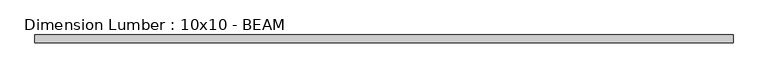
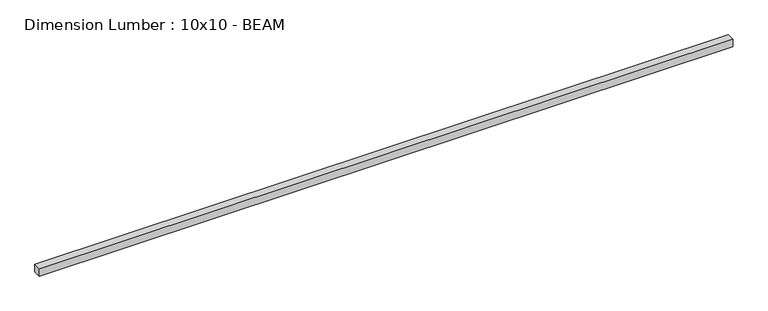
"""IFC4 building model written with IfcOpenShell, lengths in millimetres: beam geometry, Dimension Lumber : 10x10 - BEAM."""

from ifc_helpers import new_model, si_unit, frame, origin, place, context, project, spatial, polyline, outline, extrude, source, transform, mapped, element, save


def dimension_lumber_10x10_beam_47096931(model_context):
    return source(origin(), model_context, "Body", "SweptSolid", [
        extrude(outline(polyline([(10420.9864513, 117.475), (10420.9864513, -117.475), (-10420.9864513, -117.475), (-10420.9864513, 117.475), (10420.9864513, 117.475)])), frame((0.0, 0.0, -117.475), z_axis=(0.0, 0.0, 1.0), x_axis=(1.0, 0.0, 0.0)), (0.0, 0.0, 1.0), 234.95),
    ])


if __name__ == "__main__":
    model = new_model("IFC4")
    model_context = context("Model", 3, world=origin())
    ifc_project = project(units=[si_unit("LENGTHUNIT", "METRE", prefix="MILLI")], contexts=[model_context])
    site = spatial("IfcSite", under=ifc_project)
    building = spatial("IfcBuilding", under=site)
    placement = place(None, origin())
    dimension_lumber_10x10_beam_shape = dimension_lumber_10x10_beam_47096931(model_context)
    element("IfcBeam", 1, ObjectType="Dimension Lumber : 10x10 - BEAM", at=placement, inside=building, context=model_context, shape_type="MappedRepresentation", body=[
        mapped(dimension_lumber_10x10_beam_shape, transform((0.0, 0.0, 0.0), x_axis=(1.0, 0.0, 0.0), y_axis=(0.0, 1.0, 0.0), z_axis=(0.0, 0.0, 1.0))),
    ])
    save(model, "model.ifc")

# Revit data of these elements
# Type "Dimension Lumber : 10x10 - BEAM"
#   Assembly Code = "B10"
#   A = 0.0755556 SF
#   Length [instance default] = 5' - 0"
#   b = 0' - 9 1/4"
#   d = 0' - 9 1/4"
#   Structural Material = (4) CHARRED SISTERED 2X10s AT BEAM
# Element 1 (IfcBeam, "Dimension Lumber : 10x10 - BEAM")
#   Materials on its faces: "(4) CHARRED SISTERED 2X10s AT BEAM"
# Materials
#   "(4) CHARRED SISTERED 2X10s AT BEAM": class "Wood", colour RGB 144 144 144, transparency 0, Description = "Pinus Echinata", Cost = 0
